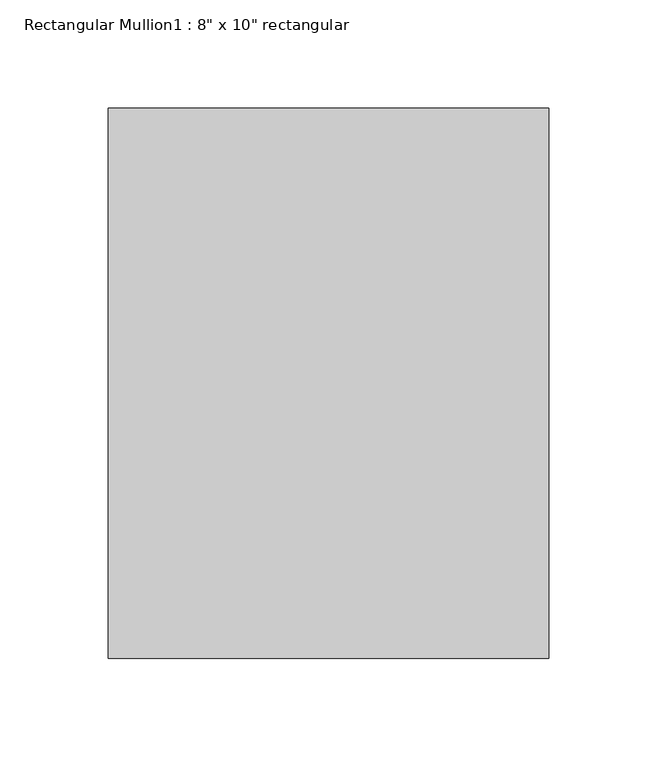
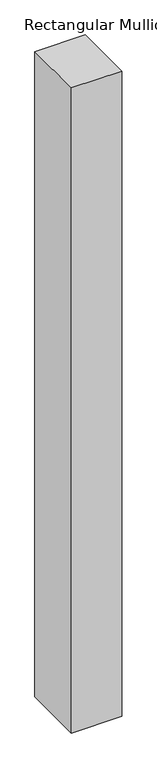
"""IFC4 building model written with IfcOpenShell, lengths in millimetres: member geometry."""

from ifc_helpers import new_model, si_unit, frame, origin, place, context, project, spatial, polyline, outline, extrude, source, transform, mapped, element, save


def member_4370fb8a(model_context):
    return source(origin(), model_context, "Body", "SweptSolid", [
        extrude(outline(polyline([(0.0, 127.0), (0.0, -127.0), (-203.2, -127.0), (-203.2, 127.0), (0.0, 127.0)])), frame((0.0, 0.0, -2743.2), z_axis=(0.0, 0.0, 1.0), x_axis=(1.0, 0.0, 0.0)), (0.0, 0.0, 1.0), 2743.2),
    ])


if __name__ == "__main__":
    model = new_model("IFC4")
    model_context = context("Model", 3, world=origin())
    ifc_project = project(units=[si_unit("LENGTHUNIT", "METRE", prefix="MILLI")], contexts=[model_context])
    site = spatial("IfcSite", under=ifc_project)
    building = spatial("IfcBuilding", under=site)
    placement = place(None, origin())
    member_shape = member_4370fb8a(model_context)
    element("IfcMember", 1, ObjectType="Rectangular Mullion1 : 8\" x 10\" rectangular", at=placement, inside=building, context=model_context, shape_type="MappedRepresentation", body=[
        mapped(member_shape, transform((0.0, 0.0, 0.0), x_axis=(1.0, 0.0, 0.0), y_axis=(0.0, 1.0, 0.0), z_axis=(0.0, 0.0, 1.0))),
    ])
    save(model, "model.ifc")

# Revit data of these elements
# Type "Rectangular Mullion1 : 8\" x 10\" rectangular"
#   built-in parameter 1007304 = 0.833333 (stored number, unit not read)
#   built-in parameter 1007301 = 0.333333 (stored number, unit not read)
#   built-in parameter 1007300 = 0.333333 (stored number, unit not read)
# Element 1 (IfcMember, "Rectangular Mullion1 : 8\" x 10\" rectangular")
#   Materials on its faces: "support-frame"
# Materials
#   "support-frame": class "Unassigned", colour RGB 233 233 233, transparency 0, Cost = 0
